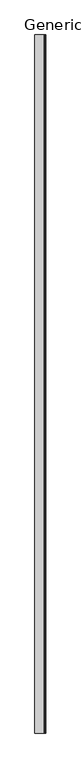
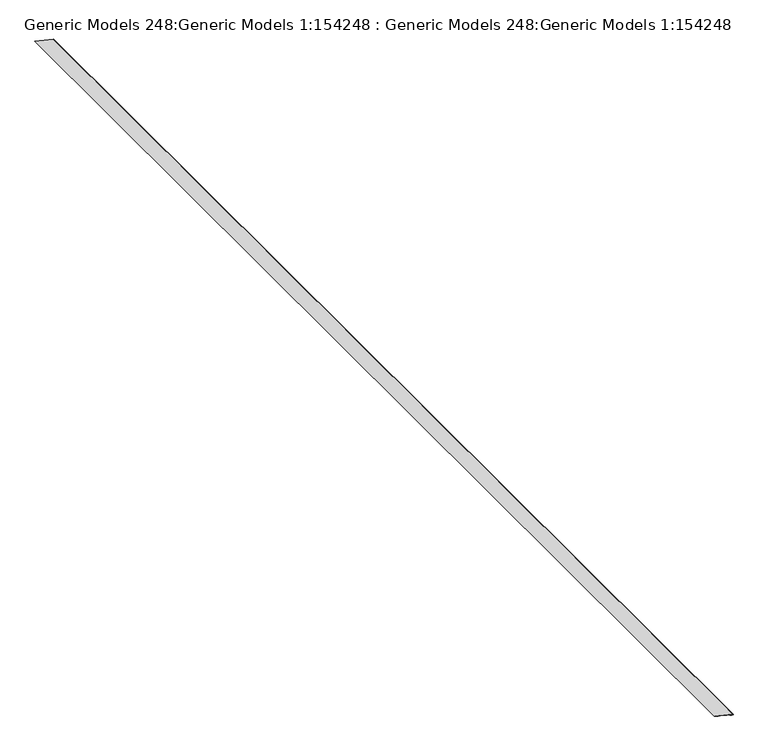
"""IFC4 building model written with IfcOpenShell, lengths in millimetres: proxy geometry, Generic Models 248:Generic Models 1:154248 : Generic Models 248:Generic Models 1:154248."""

import ifcopenshell
import ifcopenshell.guid

model = None  # the IFC model being written
_history = None  # IfcOwnerHistory: only IFC2X3 demands one
_inside = {}  # id of a spatial element -> (the spatial element, [elements in it])
_under = {}  # id of a project, library or spatial element -> (it, [spatial elements below it])
_declared = {}  # id of a project -> (the project, [libraries it declares])
_typed = {}  # id of a type object -> (the type object, [elements of that type])
_made_of = {}  # id of a material, layer set ... -> (it, [elements and type objects made of it])


def new_model(schema):
    """Start an empty IFC model of exactly this schema.

    Asked for "IFC4X3", IfcOpenShell would pick the latest addendum, in which some entities
    have other attributes; the version numbers below select the first issue.
    IFC2X3 requires an IfcOwnerHistory on every rooted entity: one is made here for all.
    """
    global model, _history
    if schema == "IFC4X3":
        model = ifcopenshell.file(schema_version=(4, 3, 0, 0))
    else:
        model = ifcopenshell.file(schema=schema)
    _inside.clear()
    _under.clear()
    _declared.clear()
    _typed.clear()
    _made_of.clear()
    _history = None
    if model.schema == "IFC2X3":
        org = make("IfcOrganization", Name="unknown")
        user = make(
            "IfcPersonAndOrganization",
            ThePerson=make("IfcPerson", FamilyName="unknown"),
            TheOrganization=org,
        )
        app = make(
            "IfcApplication",
            ApplicationDeveloper=org,
            Version="unknown",
            ApplicationFullName="unknown",
            ApplicationIdentifier="unknown",
        )
        _history = make(
            "IfcOwnerHistory",
            OwningUser=user,
            OwningApplication=app,
            ChangeAction="ADDED",
            CreationDate=0,
        )
    return model


def make(cls, **values):
    """One entity of the class cls with the attributes given. An attribute that is None is left unset."""
    return model.create_entity(
        cls, **{name: value for name, value in values.items() if value is not None}
    )


def rooted(cls, **values):
    """An entity with a GlobalId (a new one), such as an element, a storey or a relation."""
    return make(cls, GlobalId=ifcopenshell.guid.new(), OwnerHistory=_history, **values)


def si_unit(unit_type, name, prefix=None):
    """IfcSIUnit, for example si_unit("LENGTHUNIT", "METRE", prefix="MILLI")."""
    return make("IfcSIUnit", UnitType=unit_type, Prefix=prefix, Name=name)


def assignment(units):
    """IfcUnitAssignment: the units of a project."""
    return None if units is None else make("IfcUnitAssignment", Units=units)


def point(xyz):
    """IfcCartesianPoint."""
    return None if xyz is None else make("IfcCartesianPoint", Coordinates=xyz)


def direction(xyz):
    """IfcDirection."""
    return None if xyz is None else make("IfcDirection", DirectionRatios=xyz)


def frame(location, z_axis=None, x_axis=None):
    """IfcAxis2Placement3D, a coordinate frame: its origin and axes. An axis left out is left unset."""
    return make(
        "IfcAxis2Placement3D",
        Location=point(location),
        Axis=direction(z_axis),
        RefDirection=direction(x_axis),
    )


def frame_2d(location, x_axis=None):
    """IfcAxis2Placement2D, a coordinate frame in the plane: its origin and x axis."""
    return make(
        "IfcAxis2Placement2D", Location=point(location), RefDirection=direction(x_axis)
    )


def origin():
    """The frame at (0, 0, 0) with its axes left unset."""
    return frame((0.0, 0.0, 0.0))


def place(relative_to, where):
    """IfcLocalPlacement: puts the frame where relative to a parent placement (None: the world)."""
    return make(
        "IfcLocalPlacement", PlacementRelTo=relative_to, RelativePlacement=where
    )


def context(
    kind, dimensions, precision=None, world=None, true_north=None, identifier=None
):
    """IfcGeometricRepresentationContext, for example the 3D "Model" context."""
    return make(
        "IfcGeometricRepresentationContext",
        ContextIdentifier=identifier,
        ContextType=kind,
        CoordinateSpaceDimension=dimensions,
        Precision=precision,
        WorldCoordinateSystem=world,
        TrueNorth=true_north,
    )


def project(units=None, contexts=None):
    """IfcProject with its units and contexts."""
    return rooted(
        "IfcProject",
        Name="project",
        RepresentationContexts=contexts,
        UnitsInContext=assignment(units),
    )


def spatial(cls, under=None, at=None, **own):
    """A site, building, storey or space (cls), placed at a placement, below another one or the project."""
    s = rooted(cls, ObjectPlacement=at, **own)
    if under is not None:
        _under.setdefault(under.id(), (under, []))[1].append(s)
    return s


def polyline(points):
    """IfcPolyline through the points."""
    return make("IfcPolyline", Points=[point(p) for p in points])


def circle_curve(where, radius):
    """IfcCircle in the frame where."""
    return make("IfcCircle", Position=where, Radius=radius)


def trimmed(basis, trim1, trim2, sense, master):
    """IfcTrimmedCurve: the piece of a basis curve between two trims."""
    return make(
        "IfcTrimmedCurve",
        BasisCurve=basis,
        Trim1=trim1,
        Trim2=trim2,
        SenseAgreement=sense,
        MasterRepresentation=master,
    )


def segment(curve, same_sense, transition):
    """IfcCompositeCurveSegment."""
    return make(
        "IfcCompositeCurveSegment",
        Transition=transition,
        SameSense=same_sense,
        ParentCurve=curve,
    )


def composite_curve(segments, self_intersect=None):
    """IfcCompositeCurve: segments joined end to end."""
    return make("IfcCompositeCurve", Segments=segments, SelfIntersect=self_intersect)


def outline(outer, holes=None, kind="AREA"):
    """IfcArbitraryClosedProfileDef: a profile drawn as a closed curve; with holes, ...WithVoids."""
    if holes is None:
        return make("IfcArbitraryClosedProfileDef", ProfileType=kind, OuterCurve=outer)
    return make(
        "IfcArbitraryProfileDefWithVoids",
        ProfileType=kind,
        OuterCurve=outer,
        InnerCurves=holes,
    )


def extrude(swept, where, along, depth):
    """IfcExtrudedAreaSolid: the profile swept, set in the frame where, extruded along a direction by depth."""
    return make(
        "IfcExtrudedAreaSolid",
        SweptArea=swept,
        Position=where,
        ExtrudedDirection=direction(along),
        Depth=depth,
    )


def shape(context_of_items, identifier, shape_type, items):
    """IfcShapeRepresentation: the items that make up one representation, for example the "Body"."""
    return make(
        "IfcShapeRepresentation",
        ContextOfItems=context_of_items,
        RepresentationIdentifier=identifier,
        RepresentationType=shape_type,
        Items=items,
    )


def source(mapping_origin, context_of_items, identifier, shape_type, items):
    """IfcRepresentationMap: a shape defined once, which mapped items show again and again."""
    return make(
        "IfcRepresentationMap",
        MappingOrigin=mapping_origin,
        MappedRepresentation=shape(context_of_items, identifier, shape_type, items),
    )


def transform(
    local_origin,
    x_axis=None,
    y_axis=None,
    z_axis=None,
    scale=None,
    scale2=None,
    scale3=None,
    uniform=True,
):
    """IfcCartesianTransformationOperator3D, or its non-uniform kind. x_axis, y_axis, z_axis: its Axis1, 2, 3."""
    if uniform:
        return make(
            "IfcCartesianTransformationOperator3D",
            Axis1=direction(x_axis),
            Axis2=direction(y_axis),
            LocalOrigin=point(local_origin),
            Scale=scale,
            Axis3=direction(z_axis),
        )
    return make(
        "IfcCartesianTransformationOperator3DnonUniform",
        Axis1=direction(x_axis),
        Axis2=direction(y_axis),
        LocalOrigin=point(local_origin),
        Scale=scale,
        Axis3=direction(z_axis),
        Scale2=scale2,
        Scale3=scale3,
    )


def mapped(mapping_source, mapping_target):
    """IfcMappedItem: shows the shape of a source again, moved by a transform."""
    return make(
        "IfcMappedItem", MappingSource=mapping_source, MappingTarget=mapping_target
    )


def made_of(thing, what):
    """Note that an element or type object is made of a material, layer set ...; save() writes the relation."""
    if what is not None:
        _made_of.setdefault(what.id(), (what, []))[1].append(thing)
    return thing


def element(
    cls,
    number,
    at=None,
    inside=None,
    cuts=None,
    type_object=None,
    material=None,
    context=None,
    identifier="Body",
    shape_type=None,
    held_by="IfcProductDefinitionShape",
    body=None,
    shapes=None,
    **own,
):
    """One element of the class cls, such as IfcWall. Its Tag is "e" and its number.

    at: its placement. inside: the storey or other place that contains it. cuts: it is an
    opening in that element (IfcRelVoidsElement). A single representation is given by context,
    identifier, shape_type and body (its items); several are given by shapes. held_by: the class
    of the entity that holds the representations. save() writes the other relations.
    """
    e = rooted(cls, Tag="e%d" % number, ObjectPlacement=at, **own)
    if body is not None:
        shapes = [shape(context, identifier, shape_type, body)]
    if shapes is not None:
        e.Representation = make(held_by, Representations=shapes)
    if inside is not None:
        _inside.setdefault(inside.id(), (inside, []))[1].append(e)
    if cuts is not None:
        rooted(
            "IfcRelVoidsElement", RelatingBuildingElement=cuts, RelatedOpeningElement=e
        )
    if type_object is not None:
        _typed.setdefault(type_object.id(), (type_object, []))[1].append(e)
    return made_of(e, material)


def aggregate(whole, parts):
    """IfcRelAggregates: a whole, such as a stair, and the parts it consists of."""
    return rooted("IfcRelAggregates", RelatingObject=whole, RelatedObjects=parts)


def save(model, path):
    """Write the relations noted so far, then the file.

    IfcRelAggregates (storeys below a building ...), IfcRelContainedInSpatialStructure (elements
    in a storey), IfcRelDefinesByType, IfcRelAssociatesMaterial and IfcRelDeclares: one each for
    every whole, place, type object, material and project.
    """
    for whole, parts in _under.values():
        aggregate(whole, parts)
    for where, things in _inside.values():
        rooted(
            "IfcRelContainedInSpatialStructure",
            RelatedElements=things,
            RelatingStructure=where,
        )
    for kind, things in _typed.values():
        rooted("IfcRelDefinesByType", RelatedObjects=things, RelatingType=kind)
    for what, things in _made_of.values():
        rooted("IfcRelAssociatesMaterial", RelatedObjects=things, RelatingMaterial=what)
    for by, libraries in _declared.values():
        rooted("IfcRelDeclares", RelatingContext=by, RelatedDefinitions=libraries)
    model.write(path)


def generic_models_248_generic_models_1_154248_generic_models_1b80b03c(model_context):
    return source(origin(), model_context, "Body", "SweptSolid", [
        extrude(outline(composite_curve([segment(polyline([(6433.1709756, 1890.3647902), (6428.7449679, 1908.0688211)]), True, "CONTINUOUS"), segment(trimmed(circle_curve(frame_2d((6433.0196014, 1909.1374794)), 4.4061914), [point((6428.7449679, 1908.0688211))], [point((6437.294235, 1910.2061378))], False, "CARTESIAN"), True, "CONTINUOUS"), segment(polyline([(6437.294235, 1910.2061378), (6511.8487411, 1611.9881132), (6510.3086399, 1611.6030879), (6435.7541337, 1909.8211125)]), True, "CONTINUOUS"), segment(trimmed(circle_curve(frame_2d((6433.0196014, 1909.1374794)), 2.8186914), [point((6435.7541337, 1909.8211125))], [point((6430.2850691, 1908.4538464))], True, "CARTESIAN"), True, "CONTINUOUS"), segment(polyline([(6430.2850691, 1908.4538464), (6434.7110768, 1890.7498155), (6433.1709756, 1890.3647902)]), True, "CONTINUOUS")], self_intersect=False)), frame((0.0, -1800.6402746, 0.0), z_axis=(0.0, 1.0, 0.0), x_axis=(0.0, 0.0, 1.0)), (0.0, 0.0, 1.0), 19050.0),
        extrude(outline(polyline([(6439.1053239, 1888.5889207), (6434.4799864, 1878.4326568), (6438.7761978, 1861.2478112), (6437.2360966, 1860.8627859), (6432.8053469, 1878.5857844), (6437.4306844, 1888.7420482), (6433.3660477, 1905.0005951), (6434.9061489, 1905.3856204), (6439.1053239, 1888.5889207)])), frame((0.0, -1800.6402746, 0.0), z_axis=(0.0, 1.0, 0.0), x_axis=(0.0, 0.0, 1.0)), (0.0, 0.0, 1.0), 19050.0),
    ])


if __name__ == "__main__":
    model = new_model("IFC4")
    model_context = context("Model", 3, world=origin())
    ifc_project = project(units=[si_unit("LENGTHUNIT", "METRE", prefix="MILLI")], contexts=[model_context])
    site = spatial("IfcSite", under=ifc_project)
    building = spatial("IfcBuilding", under=site)
    placement = place(None, origin())
    generic_models_248_generic_models_1_154248_generic_models_shape = generic_models_248_generic_models_1_154248_generic_models_1b80b03c(model_context)
    element("IfcBuildingElementProxy", 1, Name="Generic Models 248:Generic Models 1:154248 : Generic Models 248:Generic Models 1:154248", ObjectType="Generic Models 248:Generic Models 1:154248 : Generic Models 248:Generic Models 1:154248", at=placement, inside=building, context=model_context, shape_type="MappedRepresentation", body=[
        mapped(generic_models_248_generic_models_1_154248_generic_models_shape, transform((0.0, 0.0, 0.0), x_axis=(1.0, 0.0, 0.0), y_axis=(0.0, 1.0, 0.0), z_axis=(0.0, 0.0, 1.0))),
    ])
    save(model, "model.ifc")

# Revit data of these elements
# Type "Generic Models 248:Generic Models 1:154248 : Generic Models 248:Generic Models 1:154248"
#   NameOverride = "Generic Models 248:Generic Models 1:154248"
#   ObjectTypeOverride = "Generic Models 248:Generic Models 1"
#   Reference = "Generic Models 1"
#   Category = "Generic Models"
#   Tag = "154248"
# Element 1 (IfcBuildingElementProxy, "Generic Models 248:Generic Models 1:154248 : Generic Models 248:Generic Models 1:154248")
#   Materials on its faces: "_STANDARD SEAM METAL ROOF 21413"
# Materials
#   "_STANDARD SEAM METAL ROOF 21413": class "Unassigned", colour RGB 175 175 175, transparency 0
